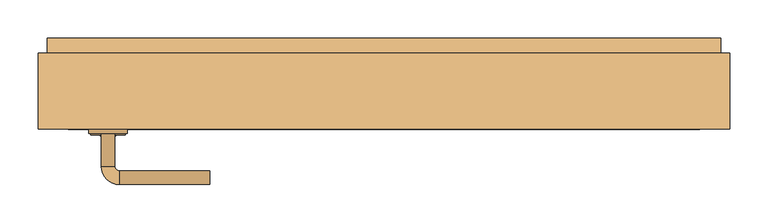
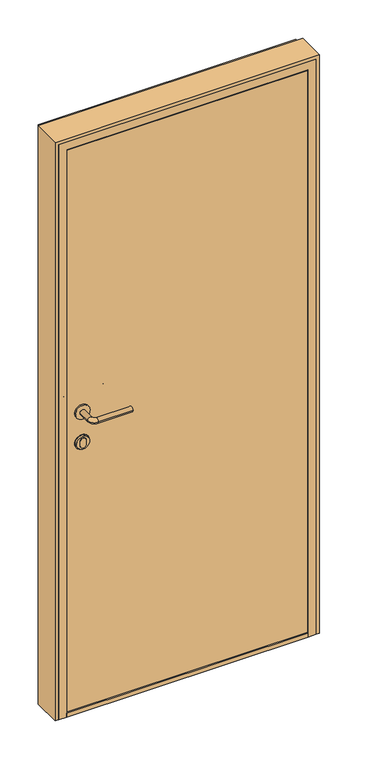
"""IFC4 building model written with IfcOpenShell, lengths in millimetres: door geometry, jeld-wen_interior_door_Stable_GW_single_1.0 : 886 x 2089 mm - M9 x M21."""

from ifc_helpers import new_model, si_unit, point, frame, origin, place, context, project, spatial, polyline, circle_curve, ellipse_curve, trimmed, outline, extrude, faceted_brep, source, transform, mapped, element, save
from ifc_brep_helpers import plane_surface, cylinder_surface, revolved_surface, advanced_brep


def door_5c2537d3(model_context):
    return source(origin(), model_context, "Body", "SolidModel", [
        advanced_brep(
        [(-385.4704625, -2.0, 983.0), (-340.4704625, -2.0, 983.0), (-371.7998782, -2.0, 995.5684608), (-372.9704625, -2.0, 991.0), (-372.9704625, -2.0, 975.0), (-363.4704625, -2.0, 965.5), (-362.4704625, -2.0, 965.5), (-352.9704625, -2.0, 975.0), (-352.9704625, -2.0, 991.0), (-362.4704625, -2.0, 1000.5), (-363.4704625, -2.0, 1000.5), (-337.9704625, -8.0, 983.0), (-387.9704625, -8.0, 983.0), (-387.9704625, -10.0, 983.0), (-337.9704625, -10.0, 983.0), (-363.4704625, -1.0, 1000.5), (-362.4704625, -1.0, 1000.5), (-352.9704625, -1.0, 991.0), (-352.9704625, -1.0, 975.0), (-362.4704625, -1.0, 965.5), (-363.4704625, -1.0, 965.5), (-372.9704625, -1.0, 975.0), (-372.9704625, -1.0, 991.0), (-371.7998782, -1.0, 995.5684608)],
        [
            (0, 1, circle_curve(frame((-362.9704625, -2.0, 983.0), z_axis=(0.0, 1.0, 0.0), x_axis=(1.0, 0.0, 0.0)), 22.5)),
            (1, 0, circle_curve(frame((-362.9704625, -2.0, 983.0), z_axis=(0.0, 1.0, 0.0), x_axis=(-1.0, 0.0, 0.0)), 22.5)),
            (2, 3, circle_curve(frame((-363.4704625, -2.0, 991.0), z_axis=(0.0, -1.0, 0.0), x_axis=(-1.0, 0.0, 0.0)), 9.5)),
            (3, 4),
            (4, 5, circle_curve(frame((-363.4704625, -2.0, 975.0), z_axis=(0.0, -1.0, 0.0), x_axis=(-1.0, 0.0, 0.0)), 9.5)),
            (5, 6),
            (6, 7, circle_curve(frame((-362.4704625, -2.0, 975.0), z_axis=(0.0, -1.0, 0.0), x_axis=(-1.0, 0.0, 0.0)), 9.5)),
            (7, 8),
            (8, 9, circle_curve(frame((-362.4704625, -2.0, 991.0), z_axis=(0.0, -1.0, 0.0), x_axis=(-1.0, 0.0, 0.0)), 9.5)),
            (9, 10),
            (10, 2, circle_curve(frame((-363.4704625, -2.0, 991.0), z_axis=(0.0, -1.0, 0.0), x_axis=(-1.0, 0.0, 0.0)), 9.5)),
            (1, 11),
            (11, 12, circle_curve(frame((-362.9704625, -8.0, 983.0), z_axis=(0.0, 1.0, 0.0), x_axis=(-1.0, 0.0, 0.0)), 25.0)),
            (12, 0),
            (12, 11, circle_curve(frame((-362.9704625, -8.0, 983.0), z_axis=(0.0, 1.0, 0.0), x_axis=(1.0, 0.0, 0.0)), 25.0)),
            (13, 14, circle_curve(frame((-362.9704625, -10.0, 983.0), z_axis=(0.0, -1.0, 0.0), x_axis=(1.0, 0.0, 0.0)), 25.0)),
            (14, 13, circle_curve(frame((-362.9704625, -10.0, 983.0), z_axis=(0.0, -1.0, 0.0), x_axis=(1.0, 0.0, 0.0)), 25.0)),
            (13, 12),
            (11, 14),
            (15, 16),
            (16, 17, circle_curve(frame((-362.4704625, -1.0, 991.0), z_axis=(0.0, 1.0, 0.0), x_axis=(-1.0, 0.0, 0.0)), 9.5)),
            (17, 18),
            (18, 19, circle_curve(frame((-362.4704625, -1.0, 975.0), z_axis=(0.0, 1.0, 0.0), x_axis=(-1.0, 0.0, 0.0)), 9.5)),
            (19, 20),
            (20, 21, circle_curve(frame((-363.4704625, -1.0, 975.0), z_axis=(0.0, 1.0, 0.0), x_axis=(-1.0, 0.0, 0.0)), 9.5)),
            (21, 22),
            (22, 23, circle_curve(frame((-363.4704625, -1.0, 991.0), z_axis=(0.0, 1.0, 0.0), x_axis=(-1.0, 0.0, 0.0)), 9.5)),
            (23, 15, circle_curve(frame((-363.4704625, -1.0, 991.0), z_axis=(0.0, 1.0, 0.0), x_axis=(-1.0, 0.0, 0.0)), 9.5)),
            (23, 2),
            (10, 15),
            (22, 3),
            (21, 4),
            (20, 5),
            (19, 6),
            (18, 7),
            (17, 8),
            (16, 9),
        ],
        [
            plane_surface(frame((-362.9704625, -2.0, 983.0), z_axis=(0.0, 1.0, 0.0), x_axis=(0.0, 0.0, -1.0))),
            revolved_surface(polyline([(-340.4704625, -2.0, 983.0), (-337.9704625, -8.0, 983.0)]), (-362.9704625, 52.0, 983.0), (0.0, -1.0, 0.0)),
            revolved_surface(polyline([(-385.4704625, -2.0, 983.0), (-387.9704625, -8.0, 983.0)]), (-362.9704625, 52.0, 983.0), (0.0, -1.0, 0.0)),
            plane_surface(frame((-337.9704625, -10.0, 983.0), z_axis=(0.0, -1.0, 0.0), x_axis=(0.0, 0.0, -1.0))),
            cylinder_surface(frame((-362.9704625, -10.0, 983.0), z_axis=(0.0, 1.0, 0.0), x_axis=(1.0, 0.0, 0.0)), 25.0),
            plane_surface(frame((-372.9704625, -1.0, 991.0), z_axis=(0.0, 1.0, 0.0), x_axis=(0.0, 0.0, -1.0))),
            cylinder_surface(frame((-363.4704625, -2.0, 991.0), z_axis=(0.0, 1.0, 0.0), x_axis=(-1.0, 0.0, 0.0)), 9.5),
            plane_surface(frame((-372.9704625, -1.0, 991.0), z_axis=(-1.0, 0.0, 0.0), x_axis=(0.0, -1.0, 0.0))),
            cylinder_surface(frame((-363.4704625, -2.0, 975.0), z_axis=(0.0, 1.0, 0.0), x_axis=(-1.0, 0.0, 0.0)), 9.5),
            plane_surface(frame((-363.4704625, -1.0, 965.5), z_axis=(0.0, 0.0, -1.0), x_axis=(0.0, -1.0, 0.0))),
            cylinder_surface(frame((-362.4704625, -2.0, 975.0), z_axis=(0.0, 1.0, 0.0), x_axis=(-1.0, 0.0, 0.0)), 9.5),
            plane_surface(frame((-352.9704625, -1.0, 975.0), z_axis=(1.0, 0.0, 0.0), x_axis=(0.0, -1.0, 0.0))),
            cylinder_surface(frame((-362.4704625, -2.0, 991.0), z_axis=(0.0, 1.0, 0.0), x_axis=(-1.0, 0.0, 0.0)), 9.5),
            plane_surface(frame((-362.4704625, -1.0, 1000.5), z_axis=(0.0, 0.0, 1.0), x_axis=(0.0, -1.0, 0.0))),
        ],
        [
            (0, [[1, 2], [3, 4, 5, 6, 7, 8, 9, 10, 11]]),
            (1, [[12, 13, 14, -2]]),
            (2, [[-14, 15, -12, -1]]),
            (3, [[16, 17]]),
            (4, [[18, -13, 19, -16]]),
            (4, [[-19, -15, -18, -17]]),
            (5, [[20, 21, 22, 23, 24, 25, 26, 27, 28]]),
            (6, [[29, -11, 30, -28]]),
            (6, [[31, -3, -29, -27]]),
            (7, [[32, -4, -31, -26]]),
            (8, [[33, -5, -32, -25]]),
            (9, [[34, -6, -33, -24]]),
            (10, [[35, -7, -34, -23]]),
            (11, [[36, -8, -35, -22]]),
            (12, [[37, -9, -36, -21]]),
            (13, [[-30, -10, -37, -20]]),
        ],
    ),
        advanced_brep(
        [(-385.4704625, -58.0, 983.0), (-340.4704625, -58.0, 983.0), (-371.7998782, -58.0, 995.5684608), (-363.4704625, -58.0, 1000.5), (-362.4704625, -58.0, 1000.5), (-352.9704625, -58.0, 991.0), (-352.9704625, -58.0, 975.0), (-362.4704625, -58.0, 965.5), (-363.4704625, -58.0, 965.5), (-372.9704625, -58.0, 975.0), (-372.9704625, -58.0, 991.0), (-387.9704625, -52.0, 983.0), (-337.9704625, -52.0, 983.0), (-387.9704625, -50.0, 983.0), (-337.9704625, -50.0, 983.0), (-363.4704625, -59.0, 1000.5), (-371.7998782, -59.0, 995.5684608), (-372.9704625, -59.0, 991.0), (-372.9704625, -59.0, 975.0), (-363.4704625, -59.0, 965.5), (-362.4704625, -59.0, 965.5), (-352.9704625, -59.0, 975.0), (-352.9704625, -59.0, 991.0), (-362.4704625, -59.0, 1000.5)],
        [
            (0, 1, circle_curve(frame((-362.9704625, -58.0, 983.0), z_axis=(0.0, -1.0, 0.0), x_axis=(-1.0, 0.0, 0.0)), 22.5)),
            (1, 0, circle_curve(frame((-362.9704625, -58.0, 983.0), z_axis=(0.0, -1.0, 0.0), x_axis=(1.0, 0.0, 0.0)), 22.5)),
            (2, 3, circle_curve(frame((-363.4704625, -58.0, 991.0), z_axis=(0.0, 1.0, 0.0), x_axis=(-1.0, 0.0, 0.0)), 9.5)),
            (3, 4),
            (4, 5, circle_curve(frame((-362.4704625, -58.0, 991.0), z_axis=(0.0, 1.0, 0.0), x_axis=(-1.0, 0.0, 0.0)), 9.5)),
            (5, 6),
            (6, 7, circle_curve(frame((-362.4704625, -58.0, 975.0), z_axis=(0.0, 1.0, 0.0), x_axis=(-1.0, 0.0, 0.0)), 9.5)),
            (7, 8),
            (8, 9, circle_curve(frame((-363.4704625, -58.0, 975.0), z_axis=(0.0, 1.0, 0.0), x_axis=(-1.0, 0.0, 0.0)), 9.5)),
            (9, 10),
            (10, 2, circle_curve(frame((-363.4704625, -58.0, 991.0), z_axis=(0.0, 1.0, 0.0), x_axis=(-1.0, 0.0, 0.0)), 9.5)),
            (0, 11),
            (11, 12, circle_curve(frame((-362.9704625, -52.0, 983.0), z_axis=(0.0, -1.0, 0.0), x_axis=(-1.0, 0.0, 0.0)), 25.0)),
            (12, 1),
            (12, 11, circle_curve(frame((-362.9704625, -52.0, 983.0), z_axis=(0.0, -1.0, 0.0), x_axis=(1.0, 0.0, 0.0)), 25.0)),
            (13, 14, circle_curve(frame((-362.9704625, -50.0, 983.0), z_axis=(0.0, 1.0, 0.0), x_axis=(1.0, 0.0, 0.0)), 25.0)),
            (14, 13, circle_curve(frame((-362.9704625, -50.0, 983.0), z_axis=(0.0, 1.0, 0.0), x_axis=(1.0, 0.0, 0.0)), 25.0)),
            (14, 12),
            (11, 13),
            (15, 16, circle_curve(frame((-363.4704625, -59.0, 991.0), z_axis=(0.0, -1.0, 0.0), x_axis=(-1.0, 0.0, 0.0)), 9.5)),
            (16, 17, circle_curve(frame((-363.4704625, -59.0, 991.0), z_axis=(0.0, -1.0, 0.0), x_axis=(-1.0, 0.0, 0.0)), 9.5)),
            (17, 18),
            (18, 19, circle_curve(frame((-363.4704625, -59.0, 975.0), z_axis=(0.0, -1.0, 0.0), x_axis=(-1.0, 0.0, 0.0)), 9.5)),
            (19, 20),
            (20, 21, circle_curve(frame((-362.4704625, -59.0, 975.0), z_axis=(0.0, -1.0, 0.0), x_axis=(-1.0, 0.0, 0.0)), 9.5)),
            (21, 22),
            (22, 23, circle_curve(frame((-362.4704625, -59.0, 991.0), z_axis=(0.0, -1.0, 0.0), x_axis=(-1.0, 0.0, 0.0)), 9.5)),
            (23, 15),
            (15, 3),
            (2, 16),
            (10, 17),
            (9, 18),
            (8, 19),
            (7, 20),
            (6, 21),
            (5, 22),
            (4, 23),
        ],
        [
            plane_surface(frame((-362.9704625, -58.0, 983.0), z_axis=(0.0, -1.0, 0.0), x_axis=(0.0, 0.0, -1.0))),
            revolved_surface(polyline([(-385.4704625, -58.0, 983.0), (-387.9704625, -52.0, 983.0)]), (-362.9704625, -112.0, 983.0), (0.0, 1.0, 0.0)),
            revolved_surface(polyline([(-340.4704625, -58.0, 983.0), (-337.9704625, -52.0, 983.0)]), (-362.9704625, -112.0, 983.0), (0.0, 1.0, 0.0)),
            plane_surface(frame((-337.9704625, -50.0, 983.0), z_axis=(0.0, 1.0, 0.0), x_axis=(0.0, 0.0, -1.0))),
            cylinder_surface(frame((-362.9704625, -50.0, 983.0), z_axis=(0.0, -1.0, 0.0), x_axis=(1.0, 0.0, 0.0)), 25.0),
            plane_surface(frame((-372.9704625, -59.0, 991.0), z_axis=(0.0, -1.0, 0.0), x_axis=(0.0, 0.0, -1.0))),
            cylinder_surface(frame((-363.4704625, -58.0, 991.0), z_axis=(0.0, -1.0, 0.0), x_axis=(-1.0, 0.0, 0.0)), 9.5),
            plane_surface(frame((-372.9704625, -59.0, 991.0), z_axis=(-1.0, 0.0, 0.0), x_axis=(0.0, 1.0, 0.0))),
            cylinder_surface(frame((-363.4704625, -58.0, 975.0), z_axis=(0.0, -1.0, 0.0), x_axis=(-1.0, 0.0, 0.0)), 9.5),
            plane_surface(frame((-363.4704625, -59.0, 965.5), z_axis=(0.0, 0.0, -1.0), x_axis=(0.0, 1.0, 0.0))),
            cylinder_surface(frame((-362.4704625, -58.0, 975.0), z_axis=(0.0, -1.0, 0.0), x_axis=(-1.0, 0.0, 0.0)), 9.5),
            plane_surface(frame((-352.9704625, -59.0, 975.0), z_axis=(1.0, 0.0, 0.0), x_axis=(0.0, 1.0, 0.0))),
            cylinder_surface(frame((-362.4704625, -58.0, 991.0), z_axis=(0.0, -1.0, 0.0), x_axis=(-1.0, 0.0, 0.0)), 9.5),
            plane_surface(frame((-362.4704625, -59.0, 1000.5), z_axis=(0.0, 0.0, 1.0), x_axis=(0.0, 1.0, 0.0))),
        ],
        [
            (0, [[1, 2], [3, 4, 5, 6, 7, 8, 9, 10, 11]]),
            (1, [[-1, 12, 13, 14]]),
            (2, [[-2, -14, 15, -12]]),
            (3, [[16, 17]]),
            (4, [[-17, 18, -13, 19]]),
            (4, [[-16, -19, -15, -18]]),
            (5, [[20, 21, 22, 23, 24, 25, 26, 27, 28]]),
            (6, [[-20, 29, -3, 30]]),
            (6, [[-21, -30, -11, 31]]),
            (7, [[-22, -31, -10, 32]]),
            (8, [[-23, -32, -9, 33]]),
            (9, [[-24, -33, -8, 34]]),
            (10, [[-25, -34, -7, 35]]),
            (11, [[-26, -35, -6, 36]]),
            (12, [[-27, -36, -5, 37]]),
            (13, [[-28, -37, -4, -29]]),
        ],
    ),
        advanced_brep(
        [(-387.9704625, -4.0, 1093.0), (-337.9704625, -4.0, 1093.0), (-354.0050698, -4.0, 1093.0), (-371.9358552, -4.0, 1093.0), (-387.9704625, -10.0, 1093.0), (-337.9704625, -10.0, 1093.0), (-354.0050698, 38.9627146, 1093.0), (-371.9358552, 38.9627146, 1093.0), (-347.9704625, 44.9973219, 1093.0), (-347.9704625, 62.9281073, 1093.0), (-228.9704625, 44.9973219, 1093.0), (-228.9704625, 62.9281073, 1093.0)],
        [
            (0, 1, circle_curve(frame((-362.9704625, -4.0, 1093.0), z_axis=(0.0, 1.0, 0.0), x_axis=(1.0, 0.0, 0.0)), 25.0)),
            (1, 0, circle_curve(frame((-362.9704625, -4.0, 1093.0), z_axis=(0.0, 1.0, 0.0), x_axis=(1.0, 0.0, 0.0)), 25.0)),
            (2, 3, circle_curve(frame((-362.9704625, -4.0, 1093.0), z_axis=(0.0, -1.0, 0.0), x_axis=(-1.0, 0.0, 0.0)), 8.9653927)),
            (3, 2, circle_curve(frame((-362.9704625, -4.0, 1093.0), z_axis=(0.0, -1.0, 0.0), x_axis=(-1.0, 0.0, 0.0)), 8.9653927)),
            (4, 5, circle_curve(frame((-362.9704625, -10.0, 1093.0), z_axis=(0.0, -1.0, 0.0), x_axis=(1.0, 0.0, 0.0)), 25.0)),
            (5, 4, circle_curve(frame((-362.9704625, -10.0, 1093.0), z_axis=(0.0, -1.0, 0.0), x_axis=(1.0, 0.0, 0.0)), 25.0)),
            (1, 5),
            (4, 0),
            (2, 6),
            (6, 7, circle_curve(frame((-362.9704625, 38.9627146, 1093.0), z_axis=(0.0, -1.0, 0.0), x_axis=(-1.0, 0.0, 0.0)), 8.9653927)),
            (7, 3),
            (7, 6, circle_curve(frame((-362.9704625, 38.9627146, 1093.0), z_axis=(0.0, -1.0, 0.0), x_axis=(-1.0, 0.0, 0.0)), 8.9653927)),
            (6, 8, circle_curve(frame((-347.9704625, 38.9627146, 1093.0), z_axis=(0.0, 0.0, -1.0), x_axis=(-1.0, 0.0, 0.0)), 6.0346073)),
            (8, 9, circle_curve(frame((-347.9704625, 53.9627146, 1093.0), z_axis=(-1.0, 0.0, 0.0), x_axis=(0.0, 1.0, 0.0)), 8.9653927)),
            (9, 7, circle_curve(frame((-347.9704625, 38.9627146, 1093.0), z_axis=(0.0, 0.0, 1.0), x_axis=(-1.0, 0.0, 0.0)), 23.9653927)),
            (9, 8, circle_curve(frame((-347.9704625, 53.9627146, 1093.0), z_axis=(-1.0, 0.0, 0.0), x_axis=(0.0, 1.0, 0.0)), 8.9653927)),
            (10, 11, circle_curve(frame((-228.9704625, 53.9627146, 1093.0), z_axis=(1.0, 0.0, 0.0), x_axis=(0.0, 1.0, 0.0)), 8.9653927)),
            (11, 10, circle_curve(frame((-228.9704625, 53.9627146, 1093.0), z_axis=(1.0, 0.0, 0.0), x_axis=(0.0, 1.0, 0.0)), 8.9653927)),
            (8, 10),
            (11, 9),
        ],
        [
            plane_surface(frame((-337.9704625, -4.0, 1093.0), z_axis=(0.0, 1.0, 0.0), x_axis=(0.0, 0.0, -1.0))),
            plane_surface(frame((-337.9704625, -10.0, 1093.0), z_axis=(0.0, -1.0, 0.0), x_axis=(0.0, 0.0, 1.0))),
            cylinder_surface(frame((-362.9704625, -4.0, 1093.0), z_axis=(0.0, -1.0, 0.0), x_axis=(1.0, 0.0, 0.0)), 25.0),
            cylinder_surface(frame((-362.9704625, -4.0, 1093.0), z_axis=(0.0, -1.0, 0.0), x_axis=(-1.0, 0.0, 0.0)), 8.9653927),
            revolved_surface(trimmed(ellipse_curve(frame((-362.9704625, 38.9627146, 1093.0), z_axis=(0.0, -1.0, 0.0), x_axis=(-1.0, 0.0, 0.0)), 8.9653927, 8.9653927), [point((-354.0050698, 38.9627146, 1093.0))], [point((-371.9358552, 38.9627146, 1093.0))], True, "CARTESIAN"), (-347.9704625, 38.9627146, 1093.0), (0.0, 0.0, -1.0)),
            revolved_surface(trimmed(ellipse_curve(frame((-362.9704625, 38.9627146, 1093.0), z_axis=(0.0, -1.0, 0.0), x_axis=(-1.0, 0.0, 0.0)), 8.9653927, 8.9653927), [point((-371.9358552, 38.9627146, 1093.0))], [point((-354.0050698, 38.9627146, 1093.0))], True, "CARTESIAN"), (-347.9704625, 38.9627146, 1093.0), (0.0, 0.0, -1.0)),
            plane_surface(frame((-228.9704625, 53.9627146, 1093.0), z_axis=(1.0, 0.0, 0.0), x_axis=(0.0, 0.0, 1.0))),
            cylinder_surface(frame((-347.9704625, 53.9627146, 1093.0), z_axis=(-1.0, 0.0, 0.0), x_axis=(0.0, 1.0, 0.0)), 8.9653927),
        ],
        [
            (0, [[1, 2], [3, 4]]),
            (1, [[5, 6]]),
            (2, [[-2, 7, -5, 8]]),
            (2, [[-1, -8, -6, -7]]),
            (3, [[9, 10, 11, -3]]),
            (3, [[-9, -4, -11, 12]]),
            (4, [[-10, 13, 14, 15]]),
            (5, [[-12, -15, 16, -13]]),
            (6, [[17, 18]]),
            (7, [[-14, 19, -18, 20]]),
            (7, [[-16, -20, -17, -19]]),
        ],
    ),
        advanced_brep(
        [(-387.9704625, -56.0, 1093.0), (-337.9704625, -56.0, 1093.0), (-354.0050698, -56.0, 1093.0), (-371.9358552, -56.0, 1093.0), (-387.9704625, -50.0, 1093.0), (-337.9704625, -50.0, 1093.0), (-371.9358552, -98.9627146, 1093.0), (-354.0050698, -98.9627146, 1093.0), (-347.9704625, -122.9281073, 1093.0), (-347.9704625, -104.9973219, 1093.0), (-228.9704625, -104.9973219, 1093.0), (-228.9704625, -122.9281073, 1093.0)],
        [
            (0, 1, circle_curve(frame((-362.9704625, -56.0, 1093.0), z_axis=(0.0, -1.0, 0.0), x_axis=(1.0, 0.0, 0.0)), 25.0)),
            (1, 0, circle_curve(frame((-362.9704625, -56.0, 1093.0), z_axis=(0.0, -1.0, 0.0), x_axis=(1.0, 0.0, 0.0)), 25.0)),
            (2, 3, circle_curve(frame((-362.9704625, -56.0, 1093.0), z_axis=(0.0, 1.0, 0.0), x_axis=(-1.0, 0.0, 0.0)), 8.9653927)),
            (3, 2, circle_curve(frame((-362.9704625, -56.0, 1093.0), z_axis=(0.0, 1.0, 0.0), x_axis=(-1.0, 0.0, 0.0)), 8.9653927)),
            (4, 5, circle_curve(frame((-362.9704625, -50.0, 1093.0), z_axis=(0.0, 1.0, 0.0), x_axis=(1.0, 0.0, 0.0)), 25.0)),
            (5, 4, circle_curve(frame((-362.9704625, -50.0, 1093.0), z_axis=(0.0, 1.0, 0.0), x_axis=(1.0, 0.0, 0.0)), 25.0)),
            (0, 4),
            (5, 1),
            (3, 6),
            (6, 7, circle_curve(frame((-362.9704625, -98.9627146, 1093.0), z_axis=(0.0, 1.0, 0.0), x_axis=(-1.0, 0.0, 0.0)), 8.9653927)),
            (7, 2),
            (7, 6, circle_curve(frame((-362.9704625, -98.9627146, 1093.0), z_axis=(0.0, 1.0, 0.0), x_axis=(-1.0, 0.0, 0.0)), 8.9653927)),
            (6, 8, circle_curve(frame((-347.9704625, -98.9627146, 1093.0), z_axis=(0.0, 0.0, 1.0), x_axis=(-1.0, 0.0, 0.0)), 23.9653927)),
            (8, 9, circle_curve(frame((-347.9704625, -113.9627146, 1093.0), z_axis=(-1.0, 0.0, 0.0), x_axis=(0.0, -1.0, 0.0)), 8.9653927)),
            (9, 7, circle_curve(frame((-347.9704625, -98.9627146, 1093.0), z_axis=(0.0, 0.0, -1.0), x_axis=(-1.0, 0.0, 0.0)), 6.0346073)),
            (9, 8, circle_curve(frame((-347.9704625, -113.9627146, 1093.0), z_axis=(-1.0, 0.0, 0.0), x_axis=(0.0, -1.0, 0.0)), 8.9653927)),
            (10, 11, circle_curve(frame((-228.9704625, -113.9627146, 1093.0), z_axis=(1.0, 0.0, 0.0), x_axis=(0.0, -1.0, 0.0)), 8.9653927)),
            (11, 10, circle_curve(frame((-228.9704625, -113.9627146, 1093.0), z_axis=(1.0, 0.0, 0.0), x_axis=(0.0, -1.0, 0.0)), 8.9653927)),
            (8, 11),
            (10, 9),
        ],
        [
            plane_surface(frame((-337.9704625, -56.0, 1093.0), z_axis=(0.0, -1.0, 0.0), x_axis=(0.0, 0.0, -1.0))),
            plane_surface(frame((-337.9704625, -50.0, 1093.0), z_axis=(0.0, 1.0, 0.0), x_axis=(0.0, 0.0, 1.0))),
            cylinder_surface(frame((-362.9704625, -56.0, 1093.0), z_axis=(0.0, 1.0, 0.0), x_axis=(1.0, 0.0, 0.0)), 25.0),
            cylinder_surface(frame((-362.9704625, -56.0, 1093.0), z_axis=(0.0, 1.0, 0.0), x_axis=(-1.0, 0.0, 0.0)), 8.9653927),
            revolved_surface(trimmed(ellipse_curve(frame((-362.9704625, -98.9627146, 1093.0), z_axis=(0.0, -1.0, 0.0), x_axis=(-1.0, 0.0, 0.0)), 8.9653927, 8.9653927), [point((-354.0050698, -98.9627146, 1093.0))], [point((-371.9358552, -98.9627146, 1093.0))], True, "CARTESIAN"), (-347.9704625, -98.9627146, 1093.0), (0.0, 0.0, -1.0)),
            revolved_surface(trimmed(ellipse_curve(frame((-362.9704625, -98.9627146, 1093.0), z_axis=(0.0, -1.0, 0.0), x_axis=(-1.0, 0.0, 0.0)), 8.9653927, 8.9653927), [point((-371.9358552, -98.9627146, 1093.0))], [point((-354.0050698, -98.9627146, 1093.0))], True, "CARTESIAN"), (-347.9704625, -98.9627146, 1093.0), (0.0, 0.0, -1.0)),
            plane_surface(frame((-228.9704625, -113.9627146, 1093.0), z_axis=(1.0, 0.0, 0.0), x_axis=(0.0, 0.0, 1.0))),
            cylinder_surface(frame((-347.9704625, -113.9627146, 1093.0), z_axis=(-1.0, 0.0, 0.0), x_axis=(0.0, -1.0, 0.0)), 8.9653927),
        ],
        [
            (0, [[1, 2], [3, 4]]),
            (1, [[5, 6]]),
            (2, [[7, -6, 8, -1]]),
            (2, [[-8, -5, -7, -2]]),
            (3, [[-4, 9, 10, 11]]),
            (3, [[12, -9, -3, -11]]),
            (4, [[13, 14, 15, -10]]),
            (5, [[-15, 16, -13, -12]]),
            (6, [[17, 18]]),
            (7, [[19, -17, 20, -14]]),
            (7, [[-20, -18, -19, -16]]),
        ],
    ),
        faceted_brep([(415.0, -50.0, 0.0), (415.0, -8.0, 0.0), (415.0, -8.0, 14.0), (415.0, -50.0, 14.0), (415.0, 50.31911, 22.0), (415.0, 36.0, 22.0), (415.0, 36.0, 0.0), (415.0, 70.0, 0.0), (415.0, 70.0, 11.7852546), (-415.0, 70.0, 0.0), (-415.0, 36.0, 0.0), (-415.0, 36.0, 22.0), (-415.0, 50.31911, 22.0), (-415.0, 70.0, 11.7852546), (-415.0, -8.0, 14.0), (-415.0, -8.0, 0.0), (-415.0, -50.0, 0.0), (-415.0, -50.0, 14.0), (403.0, 36.0, 0.0), (403.0, -8.0, 0.0), (-403.0, -8.0, 0.0), (-403.0, 36.0, 0.0), (403.0, -8.0, 14.0), (-403.0, -8.0, 14.0), (403.0, -8.0, 22.0), (-403.0, -8.0, 22.0), (-403.0, 36.0, 22.0), (403.0, 36.0, 22.0)], [[[0, 1, 2, 3]], [[4, 5, 6, 7, 8]], [[9, 10, 11, 12, 13]], [[14, 15, 16, 17]], [[7, 6, 18, 19, 1, 0, 16, 15, 20, 21, 10, 9]], [[3, 17, 16, 0]], [[2, 22, 23, 14, 17, 3]], [[23, 22, 24, 25]], [[12, 11, 26, 25, 24, 27, 5, 4]], [[8, 13, 12, 4]], [[7, 9, 13, 8]], [[20, 15, 14, 23]], [[26, 11, 10, 21]], [[23, 25, 26, 21, 20]], [[22, 2, 1, 19]], [[18, 6, 5, 27]], [[19, 18, 27, 24, 22]]]),
        extrude(outline(polyline([(412.5, -10.0), (412.5, -50.0), (-412.5, -50.0), (-412.5, -10.0), (412.5, -10.0)])), frame((0.0, 0.0, 18.0), z_axis=(0.0, 0.0, 1.0), x_axis=(1.0, 0.0, 0.0)), (0.0, 0.0, 1.0), 2040.0),
        faceted_brep([(443.0, 70.0, 0.0), (443.0, -50.0, 0.0), (415.0, -50.0, 0.0), (415.0, -8.0, 0.0), (403.0, -8.0, 0.0), (403.0, 36.0, 0.0), (415.0, 36.0, 0.0), (415.0, 70.0, 0.0), (415.0, 70.0, 2061.0), (-415.0, 70.0, 2061.0), (-415.0, 70.0, 0.0), (-443.0, 70.0, 0.0), (-443.0, 70.0, 2089.0), (443.0, 70.0, 2089.0), (415.0, 36.0, 2061.0), (403.0, 36.0, 2049.0), (-403.0, 36.0, 2049.0), (-403.0, 36.0, 0.0), (-415.0, 36.0, 0.0), (-415.0, 36.0, 2061.0), (403.0, -8.0, 2049.0), (415.0, -8.0, 2061.0), (-415.0, -8.0, 2061.0), (-415.0, -8.0, 0.0), (-403.0, -8.0, 0.0), (-403.0, -8.0, 2049.0), (415.0, -50.0, 2061.0), (443.0, -50.0, 2089.0), (-443.0, -50.0, 2089.0), (-443.0, -50.0, 0.0), (-415.0, -50.0, 0.0), (-415.0, -50.0, 2061.0)], [[[0, 1, 2, 3, 4, 5, 6, 7]], [[7, 8, 9, 10, 11, 12, 13, 0]], [[6, 14, 8, 7]], [[5, 15, 16, 17, 18, 19, 14, 6]], [[4, 20, 15, 5]], [[3, 21, 22, 23, 24, 25, 20, 4]], [[2, 26, 21, 3]], [[1, 27, 28, 29, 30, 31, 26, 2]], [[0, 13, 27, 1]], [[12, 11, 29, 28]], [[11, 10, 18, 17, 24, 23, 30, 29]], [[19, 18, 10, 9]], [[25, 24, 17, 16]], [[31, 30, 23, 22]], [[14, 19, 9, 8]], [[20, 25, 16, 15]], [[26, 31, 22, 21]], [[13, 12, 28, 27]]]),
        extrude(outline(polyline([(0.0, -443.0), (2089.0, -443.0), (2089.0, 443.0), (0.0, 443.0), (0.0, 455.0), (2101.0, 455.0), (2101.0, -455.0), (0.0, -455.0), (0.0, -443.0)])), frame((0.0, -50.0, 0.0), z_axis=(0.0, 1.0, 0.0), x_axis=(0.0, 0.0, 1.0)), (0.0, 0.0, 1.0), 100.0),
    ])


if __name__ == "__main__":
    model = new_model("IFC4")
    model_context = context("Model", 3, world=origin())
    ifc_project = project(units=[si_unit("LENGTHUNIT", "METRE", prefix="MILLI")], contexts=[model_context])
    site = spatial("IfcSite", under=ifc_project)
    building = spatial("IfcBuilding", under=site)
    placement = place(None, origin())
    door_shape = door_5c2537d3(model_context)
    element("IfcDoor", 1, ObjectType="jeld-wen_interior_door_Stable_GW_single_1.0 : 886 x 2089 mm - M9 x M21", at=placement, inside=building, context=model_context, shape_type="MappedRepresentation", body=[
        mapped(door_shape, transform((0.0, 0.0, 0.0), x_axis=(1.0, 0.0, 0.0), y_axis=(0.0, 1.0, 0.0), z_axis=(0.0, 0.0, 1.0))),
    ])
    save(model, "model.ifc")

# Revit data of these elements
# Type "jeld-wen_interior_door_Stable_GW_single_1.0 : 886 x 2089 mm - M9 x M21"
#   Type Mark = "42"
#   Youtube clip = ""
#   Uniclass 2.0 Description = "Doorsets"
#   Uniclass 2.0 Code = "PR-59-23"
#   Uniclass 1.4 Description = "Doors"
#   Uniclass 1.4 Code = "L411"
#   UNSPSC Code = "301715"
#   Technical description = "http://www.swedoor.se/mattofakta"
#   Region South America = "None"
#   Region Oceania = "None"
#   Region North America = "None"
#   Region Middle East = "None"
#   Region Europe = "DK, FI, IS, NO, SE"
#   Region Asia = "None"
#   Region Antarctica = "None"
#   Region Africa = "None"
#   QR code = "http://bimobject.com/swedoor-jeld-wen/product/int_door_stable_nature"
#   Product group = "ADVANCE-LINE - Stable Nature"
#   Product family = "Interior doors"
#   Product data url = "http://bimobject.com/swedoor-jeld-wen/product/int_door_stable_nature"
#   Product certification = "http://www.swedoor.se/goda-raad/download-center/#59360"
#   Product SKU = "int_door_stable_nature"
#   Product Guid = "2c907816-df84-4119-9f23-2aac3199c8d4"
#   NBS Reference Description = "Doorsets"
#   NBS Reference Code = "59-23"
#   Material secondary = ""
#   Material main = "Wood"
#   Manufacturer name = "SWEDOOR JELD-WEN "
#   Manufacturer country = "Denmark"
#   Manufacturer = "JELD-WEN"
#   Installation instructions = "http://www.swedoor.se/goda-raad/download-center/#6849"
#   IFC Classification = "Door"
#   EAN code = ""
#   Design country = "Denmark"
#   Date of publishing = "2015-06-11"
#   COBIe Type Category = ""
#   BIMobject category = "Doors"
#   Analytic Construction = "<None>"
#   Weight Net (Kg) = 0
#   Rough Width = 910 mm
#   Rough Height = 2101 mm
#   Nominal width = 0
#   Nominal height = 0
#   Frame Projection Ext. = 25 mm
#   Frame Projection Int. = 25 mm
#   Frame Width = 75 mm
#   Height = 2089 mm
#   Width = 886 mm
#   Frame Depth [instance default] = 120 mm
#   Door Panel Width = 825 mm
#   Door Panel Height = 2040 mm
#   Clear Opening 90° [instance default] = 760 mm
#   Standard Threshold 9 mm [instance default] = no
#   Standard Threshold 25 mm [instance default] = no
#   Standard Threshold 22 mm [instance default] = yes
#   Edition number = 1
#   Surface Material [instance default] = element 555374
#   Frame Surface Finish Material = White
#   Door Surface Finish Material = White paint
#   Function = (empty or 0)
#   Wall Closure = (empty or 0)
# Element 1 (IfcDoor, "jeld-wen_interior_door_Stable_GW_single_1.0 : 886 x 2089 mm - M9 x M21")
#   Materials on its faces: "Titanium", "White", "Wood (Oak)", "White paint"
# Materials
#   "White": class "Paint/Coating", colour RGB 250 250 250, transparency 0, Manufacturer = "Modernform", Description = "WH", Cost = 0
#   "White paint": class "Generic", colour RGB 228 228 228, transparency 0, Cost = 0
#   "Titanium": class "Metal", colour RGB 120 120 120, transparency 0, Description = "Titanium", Cost = 0
#   "Wood (Oak)": class "Wood", colour RGB 120 120 120, transparency 0, Description = "Physical material.", Cost = 0
